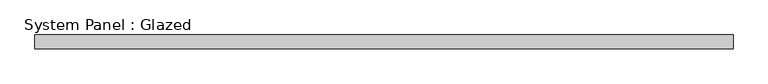
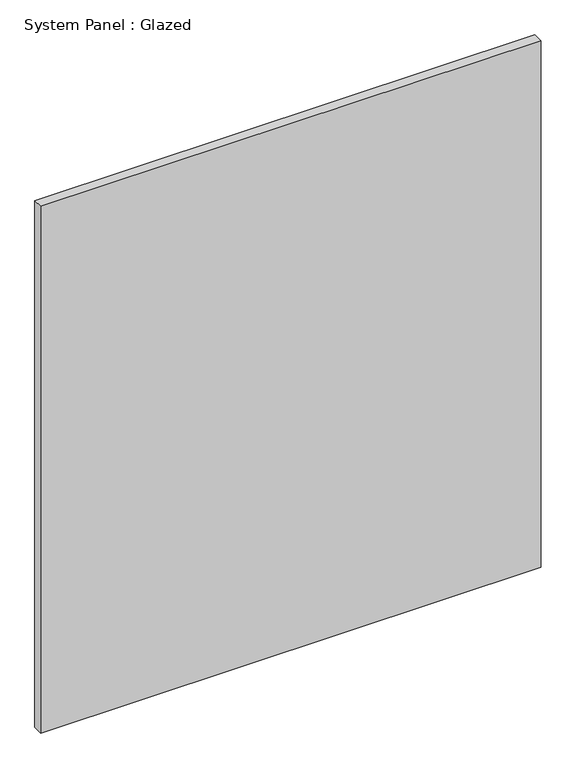
"""IFC4 building model written with IfcOpenShell, lengths in millimetres: plate geometry, System Panel : Glazed."""

from ifc_helpers import new_model, si_unit, origin, origin_with_axes, place, context, project, spatial, polyline, outline, extrude, source, transform, mapped, element, save


def system_panel_glazed_5e755b44(model_context):
    return source(origin(), model_context, "Body", "SweptSolid", [
        extrude(outline(polyline([(629.1666667, 24.5), (-629.1666667, 24.5), (-629.1666667, 49.5), (629.1666667, 49.5), (629.1666667, 24.5)])), origin_with_axes(), (0.0, 0.0, 1.0), 1400.0),
    ])


if __name__ == "__main__":
    model = new_model("IFC4")
    model_context = context("Model", 3, world=origin())
    ifc_project = project(units=[si_unit("LENGTHUNIT", "METRE", prefix="MILLI")], contexts=[model_context])
    site = spatial("IfcSite", under=ifc_project)
    building = spatial("IfcBuilding", under=site)
    placement = place(None, origin())
    system_panel_glazed_shape = system_panel_glazed_5e755b44(model_context)
    element("IfcPlate", 1, ObjectType="System Panel : Glazed", at=placement, inside=building, context=model_context, shape_type="MappedRepresentation", body=[
        mapped(system_panel_glazed_shape, transform((0.0, 0.0, 0.0), x_axis=(1.0, 0.0, 0.0), y_axis=(0.0, 1.0, 0.0), z_axis=(0.0, 0.0, 1.0))),
    ])
    save(model, "model.ifc")

# Revit data of these elements
# Element 1 (IfcPlate, "System Panel : Glazed")
#   Materials on its faces: "Glass"
# Materials
#   "Glass": class "Glass", colour RGB 0 128 192, transparency 0.9
